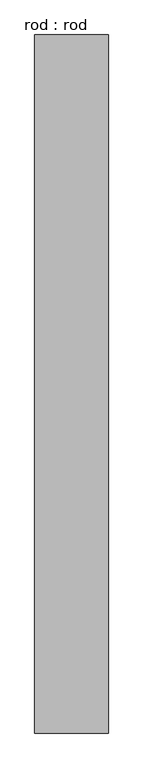
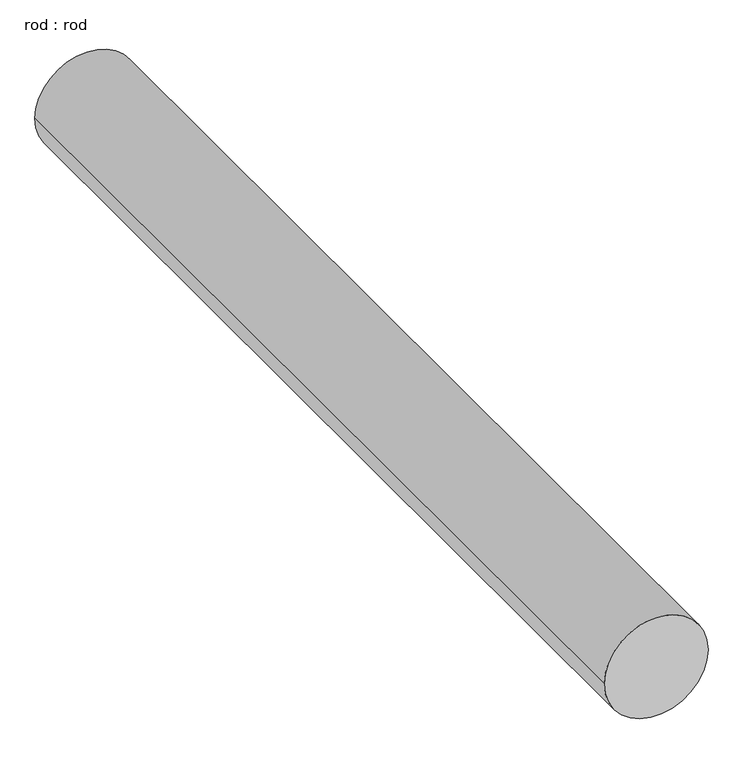
"""IFC4 building model written with IfcOpenShell, lengths in millimetres: proxy geometry, rod : rod."""

from ifc_helpers import new_model, si_unit, point, frame, frame_2d, origin, place, context, project, spatial, circle_curve, trimmed, segment, composite_curve, outline, extrude, source, transform, mapped, element, save


def rod_rod_fee6a584(model_context):
    return source(origin(), model_context, "Body", "SweptSolid", [
        extrude(outline(composite_curve([segment(trimmed(circle_curve(frame_2d((0.0108462, 0.0)), 200.0), [point((0.0108462, 200.0))], [point((0.0108462, -200.0))], False, "CARTESIAN"), True, "CONTINUOUS"), segment(trimmed(circle_curve(frame_2d((0.0108462, 0.0)), 200.0), [point((0.0108462, -200.0))], [point((0.0108462, 200.0))], False, "CARTESIAN"), True, "CONTINUOUS")], self_intersect=False)), frame((0.0, 2195.7425189, 0.0), z_axis=(0.0, 1.0, 0.0), x_axis=(0.0, 0.0, 1.0)), (0.0, 0.0, 1.0), 3793.9721928),
    ])


if __name__ == "__main__":
    model = new_model("IFC4")
    model_context = context("Model", 3, world=origin())
    ifc_project = project(units=[si_unit("LENGTHUNIT", "METRE", prefix="MILLI")], contexts=[model_context])
    site = spatial("IfcSite", under=ifc_project)
    building = spatial("IfcBuilding", under=site)
    placement = place(None, origin())
    rod_rod_shape = rod_rod_fee6a584(model_context)
    element("IfcBuildingElementProxy", 1, Name="rod : rod", ObjectType="rod : rod", at=placement, inside=building, context=model_context, shape_type="MappedRepresentation", body=[
        mapped(rod_rod_shape, transform((0.0, 0.0, 0.0), x_axis=(1.0, 0.0, 0.0), y_axis=(0.0, 1.0, 0.0), z_axis=(0.0, 0.0, 1.0))),
    ])
    save(model, "model.ifc")

# Revit data of these elements
# Type "rod : rod"
#   Default Elevation = 0
